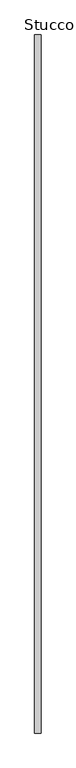
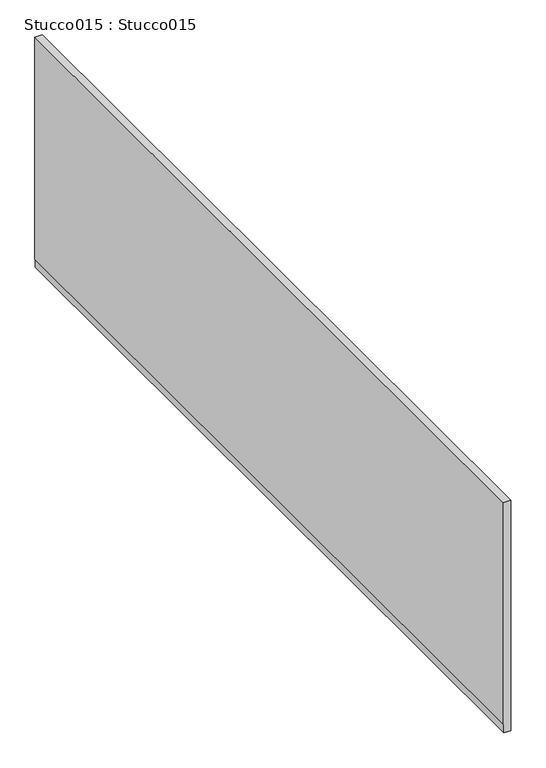
"""IFC4 building model written with IfcOpenShell, lengths in millimetres: proxy geometry, Stucco015 : Stucco015."""

from ifc_helpers import new_model, si_unit, frame, origin, place, context, project, spatial, polyline, outline, extrude, source, transform, mapped, element, save


def stucco015_stucco015_56df335f(model_context):
    return source(origin(), model_context, "Body", "SweptSolid", [
        extrude(outline(polyline([(39567.688258, -9915.4282763), (39567.688258, -9914.143256), (39545.1576447, -9914.143256), (39545.1576447, -9897.6480717), (40145.4616445, -9897.6480717), (40145.4616445, -9915.4282763), (39567.688258, -9915.4282763)])), frame((0.0, 7982.1532461, 0.0), z_axis=(0.0, 1.0, 0.0), x_axis=(0.0, 0.0, 1.0)), (0.0, 0.0, 1.0), 1999.9999999),
    ])


if __name__ == "__main__":
    model = new_model("IFC4")
    model_context = context("Model", 3, world=origin())
    ifc_project = project(units=[si_unit("LENGTHUNIT", "METRE", prefix="MILLI")], contexts=[model_context])
    site = spatial("IfcSite", under=ifc_project)
    building = spatial("IfcBuilding", under=site)
    placement = place(None, origin())
    stucco015_stucco015_shape = stucco015_stucco015_56df335f(model_context)
    element("IfcBuildingElementProxy", 1, Name="Stucco015 : Stucco015", ObjectType="Stucco015 : Stucco015", at=placement, inside=building, context=model_context, shape_type="MappedRepresentation", body=[
        mapped(stucco015_stucco015_shape, transform((0.0, 0.0, 0.0), x_axis=(1.0, 0.0, 0.0), y_axis=(0.0, 1.0, 0.0), z_axis=(0.0, 0.0, 1.0))),
    ])
    save(model, "model.ifc")

# Revit data of these elements
# Type "Stucco015 : Stucco015"
#   NameOverride = "Stucco015"
# Element 1 (IfcBuildingElementProxy, "Stucco015 : Stucco015")
#   Materials on its faces: "7/8\" SMOOTH TROWEL EXTERIOR STUCCO"
# Materials
#   "7/8\" SMOOTH TROWEL EXTERIOR STUCCO": class "Unassigned", colour RGB 255 255 255, transparency 0, Cost = 0
